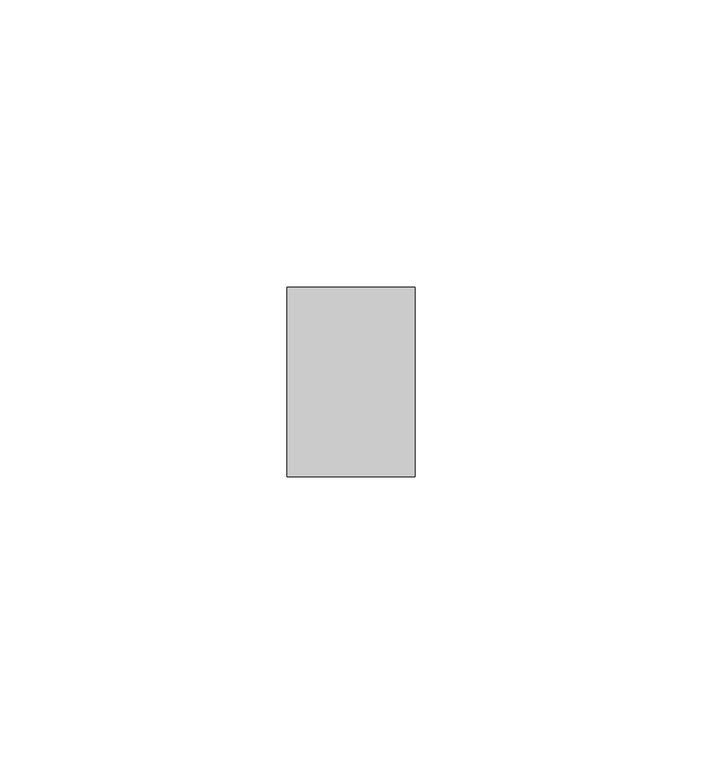
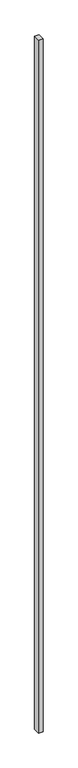
"""IFC4 building model written with IfcOpenShell, lengths in millimetres: proxy geometry, Generic Models 11:Generic Models 1:306267:Generic Models 1:306267 : Generic Models 11:Generic Models 1:306267:300405:Generic Models 1:306267:Generic Models 1:306267 : Generic Models 11:Generic Models 1:306267:300405 : Generic Models 11:Generic Models 1:306267:Generic Models 1:306267 : Generic Models 11:Generic Models 1:306267:300405:2 : Generic Models 11:Generic Models 1:306267:Generic Models 1:306267 : Generic Models 11:Generic Models 1:306267:300405:Generic Models 1:306267:Generic Models 1:306267 : Generic Models 11:Generic Models 1:306267:300405 : Generic Models 11:Generic Models 1:306267:Generic Models 1:306267 : Generic Models 11:Generic Models 1:306267:300405:300182."""

import ifcopenshell
import ifcopenshell.guid

model = None  # the IFC model being written
_history = None  # IfcOwnerHistory: only IFC2X3 demands one
_inside = {}  # id of a spatial element -> (the spatial element, [elements in it])
_under = {}  # id of a project, library or spatial element -> (it, [spatial elements below it])
_declared = {}  # id of a project -> (the project, [libraries it declares])
_typed = {}  # id of a type object -> (the type object, [elements of that type])
_made_of = {}  # id of a material, layer set ... -> (it, [elements and type objects made of it])


def new_model(schema):
    """Start an empty IFC model of exactly this schema.

    Asked for "IFC4X3", IfcOpenShell would pick the latest addendum, in which some entities
    have other attributes; the version numbers below select the first issue.
    IFC2X3 requires an IfcOwnerHistory on every rooted entity: one is made here for all.
    """
    global model, _history
    if schema == "IFC4X3":
        model = ifcopenshell.file(schema_version=(4, 3, 0, 0))
    else:
        model = ifcopenshell.file(schema=schema)
    _inside.clear()
    _under.clear()
    _declared.clear()
    _typed.clear()
    _made_of.clear()
    _history = None
    if model.schema == "IFC2X3":
        org = make("IfcOrganization", Name="unknown")
        user = make(
            "IfcPersonAndOrganization",
            ThePerson=make("IfcPerson", FamilyName="unknown"),
            TheOrganization=org,
        )
        app = make(
            "IfcApplication",
            ApplicationDeveloper=org,
            Version="unknown",
            ApplicationFullName="unknown",
            ApplicationIdentifier="unknown",
        )
        _history = make(
            "IfcOwnerHistory",
            OwningUser=user,
            OwningApplication=app,
            ChangeAction="ADDED",
            CreationDate=0,
        )
    return model


def make(cls, **values):
    """One entity of the class cls with the attributes given. An attribute that is None is left unset."""
    return model.create_entity(
        cls, **{name: value for name, value in values.items() if value is not None}
    )


def rooted(cls, **values):
    """An entity with a GlobalId (a new one), such as an element, a storey or a relation."""
    return make(cls, GlobalId=ifcopenshell.guid.new(), OwnerHistory=_history, **values)


def si_unit(unit_type, name, prefix=None):
    """IfcSIUnit, for example si_unit("LENGTHUNIT", "METRE", prefix="MILLI")."""
    return make("IfcSIUnit", UnitType=unit_type, Prefix=prefix, Name=name)


def assignment(units):
    """IfcUnitAssignment: the units of a project."""
    return None if units is None else make("IfcUnitAssignment", Units=units)


def point(xyz):
    """IfcCartesianPoint."""
    return None if xyz is None else make("IfcCartesianPoint", Coordinates=xyz)


def direction(xyz):
    """IfcDirection."""
    return None if xyz is None else make("IfcDirection", DirectionRatios=xyz)


def frame(location, z_axis=None, x_axis=None):
    """IfcAxis2Placement3D, a coordinate frame: its origin and axes. An axis left out is left unset."""
    return make(
        "IfcAxis2Placement3D",
        Location=point(location),
        Axis=direction(z_axis),
        RefDirection=direction(x_axis),
    )


def origin():
    """The frame at (0, 0, 0) with its axes left unset."""
    return frame((0.0, 0.0, 0.0))


def origin_with_axes():
    """The frame at (0, 0, 0) with the z axis (0, 0, 1) and the x axis (1, 0, 0) written out."""
    return frame((0.0, 0.0, 0.0), z_axis=(0.0, 0.0, 1.0), x_axis=(1.0, 0.0, 0.0))


def place(relative_to, where):
    """IfcLocalPlacement: puts the frame where relative to a parent placement (None: the world)."""
    return make(
        "IfcLocalPlacement", PlacementRelTo=relative_to, RelativePlacement=where
    )


def context(
    kind, dimensions, precision=None, world=None, true_north=None, identifier=None
):
    """IfcGeometricRepresentationContext, for example the 3D "Model" context."""
    return make(
        "IfcGeometricRepresentationContext",
        ContextIdentifier=identifier,
        ContextType=kind,
        CoordinateSpaceDimension=dimensions,
        Precision=precision,
        WorldCoordinateSystem=world,
        TrueNorth=true_north,
    )


def project(units=None, contexts=None):
    """IfcProject with its units and contexts."""
    return rooted(
        "IfcProject",
        Name="project",
        RepresentationContexts=contexts,
        UnitsInContext=assignment(units),
    )


def spatial(cls, under=None, at=None, **own):
    """A site, building, storey or space (cls), placed at a placement, below another one or the project."""
    s = rooted(cls, ObjectPlacement=at, **own)
    if under is not None:
        _under.setdefault(under.id(), (under, []))[1].append(s)
    return s


def polyline(points):
    """IfcPolyline through the points."""
    return make("IfcPolyline", Points=[point(p) for p in points])


def outline(outer, holes=None, kind="AREA"):
    """IfcArbitraryClosedProfileDef: a profile drawn as a closed curve; with holes, ...WithVoids."""
    if holes is None:
        return make("IfcArbitraryClosedProfileDef", ProfileType=kind, OuterCurve=outer)
    return make(
        "IfcArbitraryProfileDefWithVoids",
        ProfileType=kind,
        OuterCurve=outer,
        InnerCurves=holes,
    )


def extrude(swept, where, along, depth):
    """IfcExtrudedAreaSolid: the profile swept, set in the frame where, extruded along a direction by depth."""
    return make(
        "IfcExtrudedAreaSolid",
        SweptArea=swept,
        Position=where,
        ExtrudedDirection=direction(along),
        Depth=depth,
    )


def shape(context_of_items, identifier, shape_type, items):
    """IfcShapeRepresentation: the items that make up one representation, for example the "Body"."""
    return make(
        "IfcShapeRepresentation",
        ContextOfItems=context_of_items,
        RepresentationIdentifier=identifier,
        RepresentationType=shape_type,
        Items=items,
    )


def source(mapping_origin, context_of_items, identifier, shape_type, items):
    """IfcRepresentationMap: a shape defined once, which mapped items show again and again."""
    return make(
        "IfcRepresentationMap",
        MappingOrigin=mapping_origin,
        MappedRepresentation=shape(context_of_items, identifier, shape_type, items),
    )


def transform(
    local_origin,
    x_axis=None,
    y_axis=None,
    z_axis=None,
    scale=None,
    scale2=None,
    scale3=None,
    uniform=True,
):
    """IfcCartesianTransformationOperator3D, or its non-uniform kind. x_axis, y_axis, z_axis: its Axis1, 2, 3."""
    if uniform:
        return make(
            "IfcCartesianTransformationOperator3D",
            Axis1=direction(x_axis),
            Axis2=direction(y_axis),
            LocalOrigin=point(local_origin),
            Scale=scale,
            Axis3=direction(z_axis),
        )
    return make(
        "IfcCartesianTransformationOperator3DnonUniform",
        Axis1=direction(x_axis),
        Axis2=direction(y_axis),
        LocalOrigin=point(local_origin),
        Scale=scale,
        Axis3=direction(z_axis),
        Scale2=scale2,
        Scale3=scale3,
    )


def mapped(mapping_source, mapping_target):
    """IfcMappedItem: shows the shape of a source again, moved by a transform."""
    return make(
        "IfcMappedItem", MappingSource=mapping_source, MappingTarget=mapping_target
    )


def made_of(thing, what):
    """Note that an element or type object is made of a material, layer set ...; save() writes the relation."""
    if what is not None:
        _made_of.setdefault(what.id(), (what, []))[1].append(thing)
    return thing


def element(
    cls,
    number,
    at=None,
    inside=None,
    cuts=None,
    type_object=None,
    material=None,
    context=None,
    identifier="Body",
    shape_type=None,
    held_by="IfcProductDefinitionShape",
    body=None,
    shapes=None,
    **own,
):
    """One element of the class cls, such as IfcWall. Its Tag is "e" and its number.

    at: its placement. inside: the storey or other place that contains it. cuts: it is an
    opening in that element (IfcRelVoidsElement). A single representation is given by context,
    identifier, shape_type and body (its items); several are given by shapes. held_by: the class
    of the entity that holds the representations. save() writes the other relations.
    """
    e = rooted(cls, Tag="e%d" % number, ObjectPlacement=at, **own)
    if body is not None:
        shapes = [shape(context, identifier, shape_type, body)]
    if shapes is not None:
        e.Representation = make(held_by, Representations=shapes)
    if inside is not None:
        _inside.setdefault(inside.id(), (inside, []))[1].append(e)
    if cuts is not None:
        rooted(
            "IfcRelVoidsElement", RelatingBuildingElement=cuts, RelatedOpeningElement=e
        )
    if type_object is not None:
        _typed.setdefault(type_object.id(), (type_object, []))[1].append(e)
    return made_of(e, material)


def aggregate(whole, parts):
    """IfcRelAggregates: a whole, such as a stair, and the parts it consists of."""
    return rooted("IfcRelAggregates", RelatingObject=whole, RelatedObjects=parts)


def save(model, path):
    """Write the relations noted so far, then the file.

    IfcRelAggregates (storeys below a building ...), IfcRelContainedInSpatialStructure (elements
    in a storey), IfcRelDefinesByType, IfcRelAssociatesMaterial and IfcRelDeclares: one each for
    every whole, place, type object, material and project.
    """
    for whole, parts in _under.values():
        aggregate(whole, parts)
    for where, things in _inside.values():
        rooted(
            "IfcRelContainedInSpatialStructure",
            RelatedElements=things,
            RelatingStructure=where,
        )
    for kind, things in _typed.values():
        rooted("IfcRelDefinesByType", RelatedObjects=things, RelatingType=kind)
    for what, things in _made_of.values():
        rooted("IfcRelAssociatesMaterial", RelatedObjects=things, RelatingMaterial=what)
    for by, libraries in _declared.values():
        rooted("IfcRelDeclares", RelatingContext=by, RelatedDefinitions=libraries)
    model.write(path)


def generic_models_dfe998db(model_context):
    return source(origin(), model_context, "Body", "SweptSolid", [
        extrude(outline(polyline([(592777.8856601, -579044.4445482), (592777.8856601, -579077.4247924), (592755.6762575, -579077.4247924), (592755.6762575, -579044.4445482), (592777.8856601, -579044.4445482)])), origin_with_axes(), (0.0, 0.0, 1.0), 3689.35),
    ])


if __name__ == "__main__":
    model = new_model("IFC4")
    model_context = context("Model", 3, world=origin())
    ifc_project = project(units=[si_unit("LENGTHUNIT", "METRE", prefix="MILLI")], contexts=[model_context])
    site = spatial("IfcSite", under=ifc_project)
    building = spatial("IfcBuilding", under=site)
    placement = place(None, origin())
    generic_models_shape = generic_models_dfe998db(model_context)
    element("IfcBuildingElementProxy", 1, Name="Generic Models 11:Generic Models 1:306267:Generic Models 1:306267 : Generic Models 11:Generic Models 1:306267:300405:Generic Models 1:306267:Generic Models 1:306267 : Generic Models 11:Generic Models 1:306267:300405 : Generic Models 11:Generic Models 1:306267:Generic Models 1:306267 : Generic Models 11:Generic Models 1:306267:300405:2 : Generic Models 11:Generic Models 1:306267:Generic Models 1:306267 : Generic Models 11:Generic Models 1:306267:300405:Generic Models 1:306267:Generic Models 1:306267 : Generic Models 11:Generic Models 1:306267:300405 : Generic Models 11:Generic Models 1:306267:Generic Models 1:306267 : Generic Models 11:Generic Models 1:306267:300405:300182", ObjectType="Generic Models 11:Generic Models 1:306267:Generic Models 1:306267 : Generic Models 11:Generic Models 1:306267:300405:Generic Models 1:306267:Generic Models 1:306267 : Generic Models 11:Generic Models 1:306267:300405 : Generic Models 11:Generic Models 1:306267:Generic Models 1:306267 : Generic Models 11:Generic Models 1:306267:300405:2 : Generic Models 11:Generic Models 1:306267:Generic Models 1:306267 : Generic Models 11:Generic Models 1:306267:300405:Generic Models 1:306267:Generic Models 1:306267 : Generic Models 11:Generic Models 1:306267:300405 : Generic Models 11:Generic Models 1:306267:Generic Models 1:306267 : Generic Models 11:Generic Models 1:306267:300405:300182", at=placement, inside=building, context=model_context, shape_type="MappedRepresentation", body=[
        mapped(generic_models_shape, transform((0.0, 0.0, 0.0), x_axis=(1.0, 0.0, 0.0), y_axis=(0.0, 1.0, 0.0), z_axis=(0.0, 0.0, 1.0))),
    ])
    save(model, "model.ifc")

# Revit data of these elements
# Type "Generic Models 11:Generic Models 1:306267:Generic Models 1:306267 : Generic Models 11:Generic Models 1:306267:300405:Generic Models 1:306267:Generic Models 1:306267 : Generic Models 11:Generic Models 1:306267:300405 : Generic Models 11:Generic Models 1:306267:Generic Models 1:306267 : Generic Models 11:Generic Models 1:306267:300405:2 : Generic Models 11:Generic Models 1:306267:Generic Models 1:306267 : Generic Models 11:Generic Models 1:306267:300405:Generic Models 1:306267:Generic Models 1:306267 : Generic Models 11:Generic Models 1:306267:300405 : Generic Models 11:Generic Models 1:306267:Generic Models 1:306267 : Generic Models 11:Generic Models 1:306267:300405:300182"
#   NameOverride = "Generic Models 11:Generic Models 1:306267:Generic Models 1:306267 : Generic Models 11:Generic Models 1:306267:300405:Generic Models 1:306267:Generic Models 1:306267 : Generic Models 11:Generic Models 1:306267:300405 : Generic Models 11:Generic Models 1:306267:Generic Models 1:306267 : Generic Models 11:Generic Models 1:306267:300405:300182"
#   ObjectTypeOverride = "Generic Models 1:306267:Generic Models 1:306267 : Generic Models 11:Generic Models 1:306267:300405 : Generic Models 11:Generic Models 1:306267:Generic Models 1:306267 : Generic Models 11:Generic Models 1:306267:300405"
#   Reference = "Generic Models 1"
#   Tag = "300182"
# Element 1 (IfcBuildingElementProxy, "Generic Models 11:Generic Models 1:306267:Generic Models 1:306267 : Generic Models 11:Generic Models 1:306267:300405:Generic Models 1:306267:Generic Models 1:306267 : Generic Models 11:Generic Models 1:306267:300405 : Generic Models 11:Generic Models 1:306267:Generic Models 1:306267 : Generic Models 11:Generic Models 1:306267:300405:2 : Generic Models 11:Generic Models 1:306267:Generic Models 1:306267 : Generic Models 11:Generic Models 1:306267:300405:Generic Models 1:306267:Generic Models 1:306267 : Generic Models 11:Generic Models 1:306267:300405 : Generic Models 11:Generic Models 1:306267:Generic Models 1:306267 : Generic Models 11:Generic Models 1:306267:300405:300182")
#   Materials on its faces: "LOW VOLUMN EXPANDABLE FOAM INSULATION"
# Materials
#   "LOW VOLUMN EXPANDABLE FOAM INSULATION": class "Unassigned", colour RGB 213 216 95, transparency 0, Cost = 0
